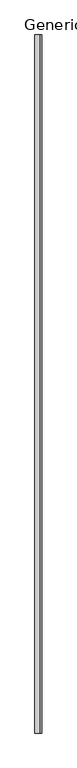
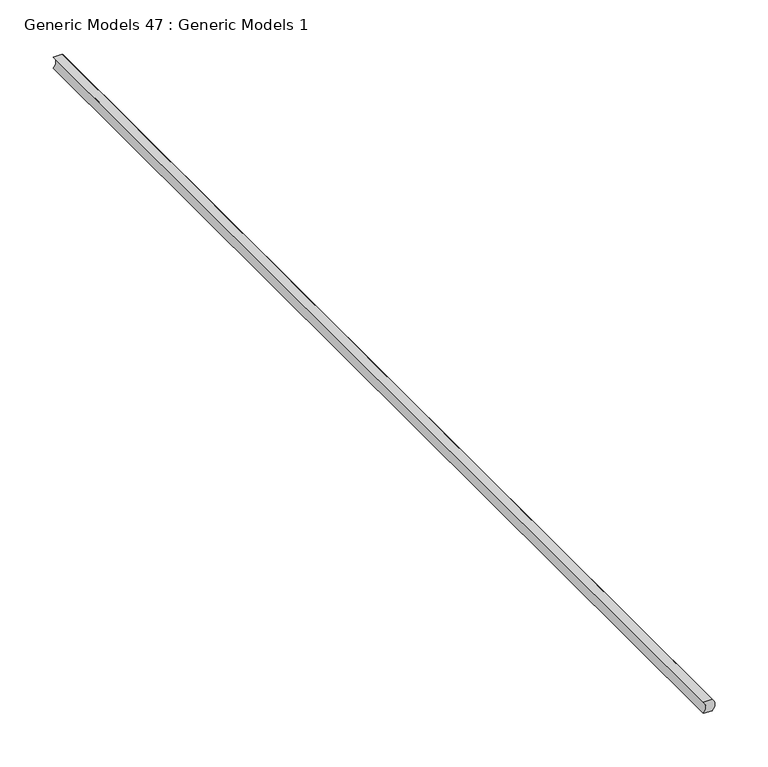
"""IFC4 building model written with IfcOpenShell, lengths in millimetres: proxy geometry, Generic Models 47 : Generic Models 1."""

from ifc_helpers import new_model, si_unit, point, frame, frame_2d, origin, place, context, project, spatial, polyline, circle_curve, trimmed, segment, composite_curve, outline, extrude, source, transform, mapped, element, save


def generic_models_47_generic_models_1_9e68d635(model_context):
    return source(origin(), model_context, "Body", "SweptSolid", [
        extrude(outline(composite_curve([segment(polyline([(2438.4, 50759.2377541), (2438.4, 50768.7627541)]), True, "CONTINUOUS"), segment(trimmed(circle_curve(frame_2d((2444.75, 50762.9332731)), 8.620055), [point((2438.4, 50768.7627541))], [point((2451.1, 50768.7627541))], False, "CARTESIAN"), True, "CONTINUOUS"), segment(polyline([(2451.1, 50768.7627541), (2451.1, 50759.2377541)]), True, "CONTINUOUS"), segment(trimmed(circle_curve(frame_2d((2444.75, 50753.4082731)), 8.620055), [point((2451.1, 50759.2377541))], [point((2438.4, 50759.2377541))], True, "CARTESIAN"), True, "CONTINUOUS")], self_intersect=False)), frame((0.0, 0.0, 0.0), z_axis=(0.0, 1.0, 0.0), x_axis=(0.0, 0.0, 1.0)), (0.0, 0.0, 1.0), 1219.2),
    ])


if __name__ == "__main__":
    model = new_model("IFC4")
    model_context = context("Model", 3, world=origin())
    ifc_project = project(units=[si_unit("LENGTHUNIT", "METRE", prefix="MILLI")], contexts=[model_context])
    site = spatial("IfcSite", under=ifc_project)
    building = spatial("IfcBuilding", under=site)
    placement = place(None, origin())
    generic_models_47_generic_models_1_shape = generic_models_47_generic_models_1_9e68d635(model_context)
    element("IfcBuildingElementProxy", 1, Name="Generic Models 47 : Generic Models 1", ObjectType="Generic Models 47 : Generic Models 1", at=placement, inside=building, context=model_context, shape_type="MappedRepresentation", body=[
        mapped(generic_models_47_generic_models_1_shape, transform((0.0, 0.0, 0.0), x_axis=(1.0, 0.0, 0.0), y_axis=(0.0, 1.0, 0.0), z_axis=(0.0, 0.0, 1.0))),
    ])
    save(model, "model.ifc")

# Revit data of these elements
# Element 1 (IfcBuildingElementProxy, "Generic Models 47 : Generic Models 1")
#   Materials on its faces: "ACOUSTICAL SEALANT"
# Materials
#   "ACOUSTICAL SEALANT": class "Unassigned", colour RGB 120 120 120, transparency 0, Cost = 0
